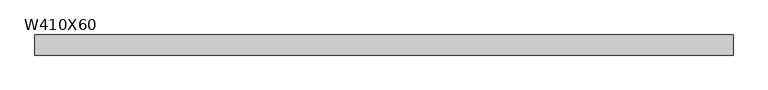
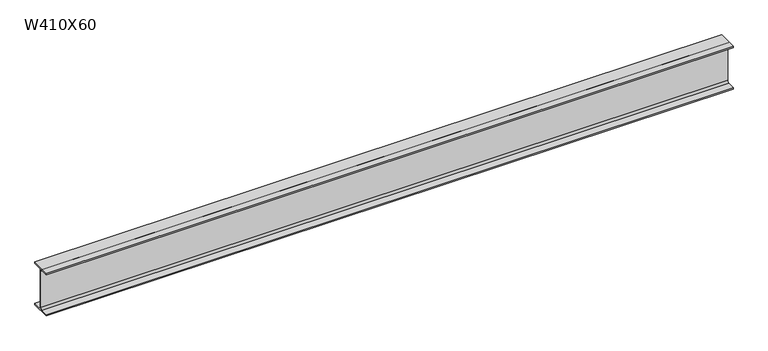
"""IFC4 building model written with IfcOpenShell, lengths in millimetres: beam geometry, M_W-Wide Flange : W410X60."""

from ifc_helpers import new_model, si_unit, point, frame, frame_2d, origin, place, context, project, spatial, polyline, circle_curve, trimmed, segment, composite_curve, outline, extrude, source, transform, mapped, element, save


def w410x60_94aca3fc(model_context):
    return source(origin(), model_context, "Body", "SweptSolid", [
        extrude(outline(composite_curve([segment(polyline([(89.0, -190.7), (89.0, -203.5), (-89.0, -203.5), (-89.0, -190.7), (-21.05, -190.7)]), True, "CONTINUOUS"), segment(trimmed(circle_curve(frame_2d((-21.05, -173.5)), 17.2), [point((-21.05, -190.7))], [point((-3.85, -173.5))], True, "CARTESIAN"), True, "CONTINUOUS"), segment(polyline([(-3.85, -173.5), (-3.85, 173.5)]), True, "CONTINUOUS"), segment(trimmed(circle_curve(frame_2d((-21.05, 173.5)), 17.2), [point((-3.85, 173.5))], [point((-21.05, 190.7))], True, "CARTESIAN"), True, "CONTINUOUS"), segment(polyline([(-21.05, 190.7), (-89.0, 190.7), (-89.0, 203.5), (89.0, 203.5), (89.0, 190.7), (21.05, 190.7)]), True, "CONTINUOUS"), segment(trimmed(circle_curve(frame_2d((21.05, 173.5)), 17.2), [point((21.05, 190.7))], [point((3.85, 173.5))], True, "CARTESIAN"), True, "CONTINUOUS"), segment(polyline([(3.85, 173.5), (3.85, -173.5)]), True, "CONTINUOUS"), segment(trimmed(circle_curve(frame_2d((21.05, -173.5)), 17.2), [point((3.85, -173.5))], [point((21.05, -190.7))], True, "CARTESIAN"), True, "CONTINUOUS"), segment(polyline([(21.05, -190.7), (89.0, -190.7)]), True, "CONTINUOUS")], self_intersect=False)), frame((-3090.9435602, 0.0, 0.0), z_axis=(1.0, 0.0, 0.0), x_axis=(0.0, 1.0, 0.0)), (0.0, 0.0, 1.0), 6181.8871204),
    ])


if __name__ == "__main__":
    model = new_model("IFC4")
    model_context = context("Model", 3, world=origin())
    ifc_project = project(units=[si_unit("LENGTHUNIT", "METRE", prefix="MILLI")], contexts=[model_context])
    site = spatial("IfcSite", under=ifc_project)
    building = spatial("IfcBuilding", under=site)
    placement = place(None, origin())
    w410x60_shape = w410x60_94aca3fc(model_context)
    element("IfcBeam", 1, ObjectType="M_W-Wide Flange : W410X60", at=placement, inside=building, context=model_context, shape_type="MappedRepresentation", body=[
        mapped(w410x60_shape, transform((0.0, 0.0, 0.0), x_axis=(1.0, 0.0, 0.0), y_axis=(0.0, 1.0, 0.0), z_axis=(0.0, 0.0, 1.0))),
    ])
    save(model, "model.ifc")

# Revit data of these elements
# Type "M_W-Wide Flange : W410X60"
#   Manufacturer = "Manufacturer"
#   AccessibilityPerformance = "AccessibilityPerformance"
#   CodePerformance = "CodePerformance"
#   Color = "Color"
#   Constituents = "Constituents"
#   Features = "Features"
#   Finish = "Finish"
#   Grade = "Grade"
#   Material = "Material"
#   ModelReference = "ModelReference"
#   NominalHeight = "NominalHeight"
#   NominalLength = "NominalLength"
#   NominalWidth = "NominalWidth"
#   ProductionYear = "ProductionYear"
#   Reference = "Reference"
#   Shape = "Shape"
#   Size = "Size"
#   SustainabilityPerformance = "SustainabilityPerformance"
#   WarrantyDescription = "WarrantyDescription"
#   WarrantyDurationLabor = "WarrantyDurationLabor"
#   WarrantyDurationParts = "WarrantyDurationParts"
#   WarrantyGuarantorLabor = "WarrantyGuarantorLabor"
#   WarrantyGuarantorParts = "WarrantyGuarantorParts"
#   ExpectedLife = "ExpectedLife"
#   ReplacementCost = "ReplacementCost"
#   AssetAccountingType = "FIXED"
#   ModelLabel = "ModelLabel"
#   W = 0.58
#   Start Extension Calculation [instance default] = 3.000 m
#   Start Extension [instance default] = -0.0127 m
#   End Extension Calculation [instance default] = 3.000 m
#   End Extension [instance default] = -0.0127 m
#   Length [instance default] = 1.524 m
#   bf = 0.178 m
#   d = 0.407 m
#   k = 0.030 m
#   kr = 0.0172 m
#   tf = 0.0128 m
#   tw = 0.0077 m
#   A = 0.0076 m²
#   Structural Material [instance default] = Metal - Steel - 345 MPa
#   Assembly Code = ""
# Element 1 (IfcBeam, "M_W-Wide Flange : W410X60")
#   Materials on its faces: "Metal - Steel - 345 MPa"
# Materials
#   "Metal - Steel - 345 MPa": class "Metal", colour RGB 247 247 247, transparency 0
